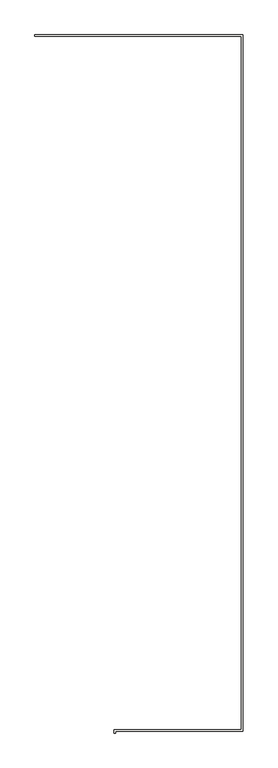
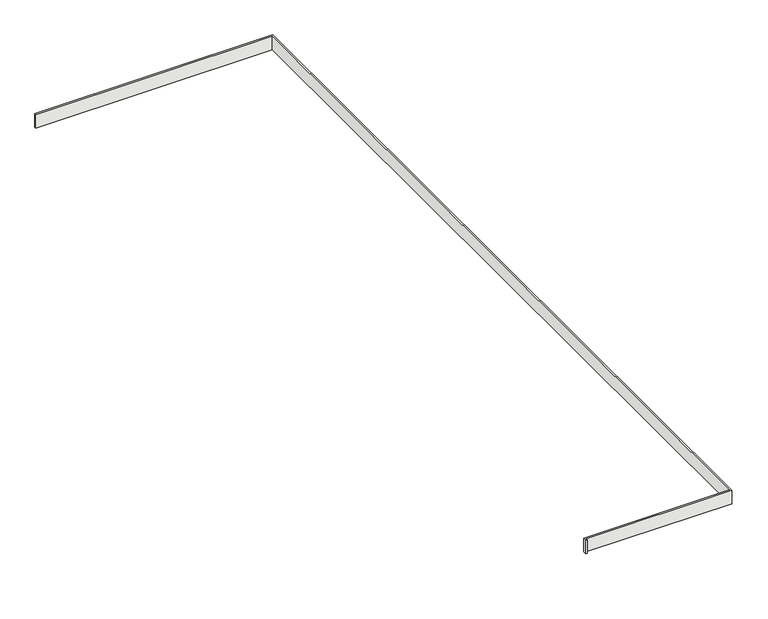
"""IFC4 building model written with IfcOpenShell, lengths in millimetres: slab geometry, FECHAMENTO DECK DE MADEIRA1 : CC_ND 300 FECHAMENTO 2 x 18 cm DECK DE MADEIRA."""

import ifcopenshell
import ifcopenshell.guid

model = None  # the IFC model being written
_history = None  # IfcOwnerHistory: only IFC2X3 demands one
_inside = {}  # id of a spatial element -> (the spatial element, [elements in it])
_under = {}  # id of a project, library or spatial element -> (it, [spatial elements below it])
_declared = {}  # id of a project -> (the project, [libraries it declares])
_typed = {}  # id of a type object -> (the type object, [elements of that type])
_made_of = {}  # id of a material, layer set ... -> (it, [elements and type objects made of it])


def new_model(schema):
    """Start an empty IFC model of exactly this schema.

    Asked for "IFC4X3", IfcOpenShell would pick the latest addendum, in which some entities
    have other attributes; the version numbers below select the first issue.
    IFC2X3 requires an IfcOwnerHistory on every rooted entity: one is made here for all.
    """
    global model, _history
    if schema == "IFC4X3":
        model = ifcopenshell.file(schema_version=(4, 3, 0, 0))
    else:
        model = ifcopenshell.file(schema=schema)
    _inside.clear()
    _under.clear()
    _declared.clear()
    _typed.clear()
    _made_of.clear()
    _history = None
    if model.schema == "IFC2X3":
        org = make("IfcOrganization", Name="unknown")
        user = make(
            "IfcPersonAndOrganization",
            ThePerson=make("IfcPerson", FamilyName="unknown"),
            TheOrganization=org,
        )
        app = make(
            "IfcApplication",
            ApplicationDeveloper=org,
            Version="unknown",
            ApplicationFullName="unknown",
            ApplicationIdentifier="unknown",
        )
        _history = make(
            "IfcOwnerHistory",
            OwningUser=user,
            OwningApplication=app,
            ChangeAction="ADDED",
            CreationDate=0,
        )
    return model


def make(cls, **values):
    """One entity of the class cls with the attributes given. An attribute that is None is left unset."""
    return model.create_entity(
        cls, **{name: value for name, value in values.items() if value is not None}
    )


def rooted(cls, **values):
    """An entity with a GlobalId (a new one), such as an element, a storey or a relation."""
    return make(cls, GlobalId=ifcopenshell.guid.new(), OwnerHistory=_history, **values)


def si_unit(unit_type, name, prefix=None):
    """IfcSIUnit, for example si_unit("LENGTHUNIT", "METRE", prefix="MILLI")."""
    return make("IfcSIUnit", UnitType=unit_type, Prefix=prefix, Name=name)


def assignment(units):
    """IfcUnitAssignment: the units of a project."""
    return None if units is None else make("IfcUnitAssignment", Units=units)


def point(xyz):
    """IfcCartesianPoint."""
    return None if xyz is None else make("IfcCartesianPoint", Coordinates=xyz)


def direction(xyz):
    """IfcDirection."""
    return None if xyz is None else make("IfcDirection", DirectionRatios=xyz)


def frame(location, z_axis=None, x_axis=None):
    """IfcAxis2Placement3D, a coordinate frame: its origin and axes. An axis left out is left unset."""
    return make(
        "IfcAxis2Placement3D",
        Location=point(location),
        Axis=direction(z_axis),
        RefDirection=direction(x_axis),
    )


def origin():
    """The frame at (0, 0, 0) with its axes left unset."""
    return frame((0.0, 0.0, 0.0))


def place(relative_to, where):
    """IfcLocalPlacement: puts the frame where relative to a parent placement (None: the world)."""
    return make(
        "IfcLocalPlacement", PlacementRelTo=relative_to, RelativePlacement=where
    )


def context(
    kind, dimensions, precision=None, world=None, true_north=None, identifier=None
):
    """IfcGeometricRepresentationContext, for example the 3D "Model" context."""
    return make(
        "IfcGeometricRepresentationContext",
        ContextIdentifier=identifier,
        ContextType=kind,
        CoordinateSpaceDimension=dimensions,
        Precision=precision,
        WorldCoordinateSystem=world,
        TrueNorth=true_north,
    )


def project(units=None, contexts=None):
    """IfcProject with its units and contexts."""
    return rooted(
        "IfcProject",
        Name="project",
        RepresentationContexts=contexts,
        UnitsInContext=assignment(units),
    )


def spatial(cls, under=None, at=None, **own):
    """A site, building, storey or space (cls), placed at a placement, below another one or the project."""
    s = rooted(cls, ObjectPlacement=at, **own)
    if under is not None:
        _under.setdefault(under.id(), (under, []))[1].append(s)
    return s


def polyline(points):
    """IfcPolyline through the points."""
    return make("IfcPolyline", Points=[point(p) for p in points])


def outline(outer, holes=None, kind="AREA"):
    """IfcArbitraryClosedProfileDef: a profile drawn as a closed curve; with holes, ...WithVoids."""
    if holes is None:
        return make("IfcArbitraryClosedProfileDef", ProfileType=kind, OuterCurve=outer)
    return make(
        "IfcArbitraryProfileDefWithVoids",
        ProfileType=kind,
        OuterCurve=outer,
        InnerCurves=holes,
    )


def extrude(swept, where, along, depth):
    """IfcExtrudedAreaSolid: the profile swept, set in the frame where, extruded along a direction by depth."""
    return make(
        "IfcExtrudedAreaSolid",
        SweptArea=swept,
        Position=where,
        ExtrudedDirection=direction(along),
        Depth=depth,
    )


def shape(context_of_items, identifier, shape_type, items):
    """IfcShapeRepresentation: the items that make up one representation, for example the "Body"."""
    return make(
        "IfcShapeRepresentation",
        ContextOfItems=context_of_items,
        RepresentationIdentifier=identifier,
        RepresentationType=shape_type,
        Items=items,
    )


def source(mapping_origin, context_of_items, identifier, shape_type, items):
    """IfcRepresentationMap: a shape defined once, which mapped items show again and again."""
    return make(
        "IfcRepresentationMap",
        MappingOrigin=mapping_origin,
        MappedRepresentation=shape(context_of_items, identifier, shape_type, items),
    )


def transform(
    local_origin,
    x_axis=None,
    y_axis=None,
    z_axis=None,
    scale=None,
    scale2=None,
    scale3=None,
    uniform=True,
):
    """IfcCartesianTransformationOperator3D, or its non-uniform kind. x_axis, y_axis, z_axis: its Axis1, 2, 3."""
    if uniform:
        return make(
            "IfcCartesianTransformationOperator3D",
            Axis1=direction(x_axis),
            Axis2=direction(y_axis),
            LocalOrigin=point(local_origin),
            Scale=scale,
            Axis3=direction(z_axis),
        )
    return make(
        "IfcCartesianTransformationOperator3DnonUniform",
        Axis1=direction(x_axis),
        Axis2=direction(y_axis),
        LocalOrigin=point(local_origin),
        Scale=scale,
        Axis3=direction(z_axis),
        Scale2=scale2,
        Scale3=scale3,
    )


def mapped(mapping_source, mapping_target):
    """IfcMappedItem: shows the shape of a source again, moved by a transform."""
    return make(
        "IfcMappedItem", MappingSource=mapping_source, MappingTarget=mapping_target
    )


def made_of(thing, what):
    """Note that an element or type object is made of a material, layer set ...; save() writes the relation."""
    if what is not None:
        _made_of.setdefault(what.id(), (what, []))[1].append(thing)
    return thing


def element(
    cls,
    number,
    at=None,
    inside=None,
    cuts=None,
    type_object=None,
    material=None,
    context=None,
    identifier="Body",
    shape_type=None,
    held_by="IfcProductDefinitionShape",
    body=None,
    shapes=None,
    **own,
):
    """One element of the class cls, such as IfcWall. Its Tag is "e" and its number.

    at: its placement. inside: the storey or other place that contains it. cuts: it is an
    opening in that element (IfcRelVoidsElement). A single representation is given by context,
    identifier, shape_type and body (its items); several are given by shapes. held_by: the class
    of the entity that holds the representations. save() writes the other relations.
    """
    e = rooted(cls, Tag="e%d" % number, ObjectPlacement=at, **own)
    if body is not None:
        shapes = [shape(context, identifier, shape_type, body)]
    if shapes is not None:
        e.Representation = make(held_by, Representations=shapes)
    if inside is not None:
        _inside.setdefault(inside.id(), (inside, []))[1].append(e)
    if cuts is not None:
        rooted(
            "IfcRelVoidsElement", RelatingBuildingElement=cuts, RelatedOpeningElement=e
        )
    if type_object is not None:
        _typed.setdefault(type_object.id(), (type_object, []))[1].append(e)
    return made_of(e, material)


def aggregate(whole, parts):
    """IfcRelAggregates: a whole, such as a stair, and the parts it consists of."""
    return rooted("IfcRelAggregates", RelatingObject=whole, RelatedObjects=parts)


def save(model, path):
    """Write the relations noted so far, then the file.

    IfcRelAggregates (storeys below a building ...), IfcRelContainedInSpatialStructure (elements
    in a storey), IfcRelDefinesByType, IfcRelAssociatesMaterial and IfcRelDeclares: one each for
    every whole, place, type object, material and project.
    """
    for whole, parts in _under.values():
        aggregate(whole, parts)
    for where, things in _inside.values():
        rooted(
            "IfcRelContainedInSpatialStructure",
            RelatedElements=things,
            RelatingStructure=where,
        )
    for kind, things in _typed.values():
        rooted("IfcRelDefinesByType", RelatedObjects=things, RelatingType=kind)
    for what, things in _made_of.values():
        rooted("IfcRelAssociatesMaterial", RelatedObjects=things, RelatingMaterial=what)
    for by, libraries in _declared.values():
        rooted("IfcRelDeclares", RelatingContext=by, RelatedDefinitions=libraries)
    model.write(path)


def slab_ccd32a31(model_context):
    return source(origin(), model_context, "Body", "SweptSolid", [
        extrude(outline(polyline([(11009.718693, -4345.5699847), (10989.718693, -4345.5699847), (10989.718693, -4295.5699847), (12839.718693, -4295.5699847), (12839.718693, 5754.4300153), (9839.718693, 5754.4300153), (9839.718693, 5774.4300153), (12859.718693, 5774.4300153), (12859.718693, -4315.5699847), (11009.718693, -4315.5699847), (11009.718693, -4345.5699847)])), frame((0.0, 0.0, 200.0), z_axis=(0.0, 0.0, 1.0), x_axis=(1.0, 0.0, 0.0)), (0.0, 0.0, 1.0), 180.0),
    ])


if __name__ == "__main__":
    model = new_model("IFC4")
    model_context = context("Model", 3, world=origin())
    ifc_project = project(units=[si_unit("LENGTHUNIT", "METRE", prefix="MILLI")], contexts=[model_context])
    site = spatial("IfcSite", under=ifc_project)
    building = spatial("IfcBuilding", under=site)
    placement = place(None, origin())
    slab_shape = slab_ccd32a31(model_context)
    element("IfcSlab", 1, ObjectType="FECHAMENTO DECK DE MADEIRA1 : CC_ND 300 FECHAMENTO 2 x 18 cm DECK DE MADEIRA", at=placement, inside=building, context=model_context, shape_type="MappedRepresentation", body=[
        mapped(slab_shape, transform((0.0, 0.0, 0.0), x_axis=(1.0, 0.0, 0.0), y_axis=(0.0, 1.0, 0.0), z_axis=(0.0, 0.0, 1.0))),
    ])
    save(model, "model.ifc")

# Revit data of these elements
# Element 1 (IfcSlab, "FECHAMENTO DECK DE MADEIRA1 : CC_ND 300 FECHAMENTO 2 x 18 cm DECK DE MADEIRA")
#   Materials on its faces: ".DECK DE MADEIRA LONGITUDINAL"
# Materials
#   ".DECK DE MADEIRA LONGITUDINAL": class ".CC_MADEIRA REVEST.", colour RGB 169 114 85, transparency 0, Description = "Deck de madeira", Cost = 0
